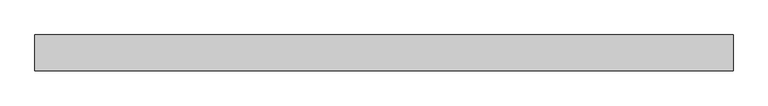
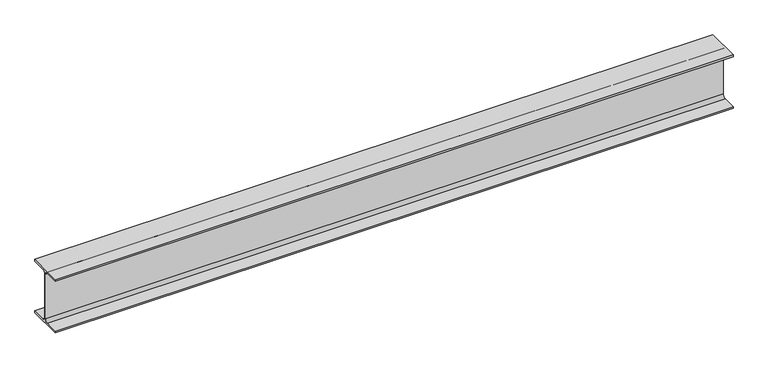
"""IFC4 building model written with IfcOpenShell, lengths in millimetres: beam geometry, 0912_Steel Framing_H-KSD3502 : H_SB_ASB_H-482x300x11x15."""

from ifc_helpers import new_model, si_unit, point, frame, frame_2d, origin, place, context, project, spatial, polyline, circle_curve, trimmed, segment, composite_curve, outline, extrude, source, transform, mapped, element, save


def beam_f33ae538(model_context):
    return source(origin(), model_context, "Body", "SweptSolid", [
        extrude(outline(composite_curve([segment(polyline([(150.0, -226.0), (150.0, -241.0), (-150.0, -241.0), (-150.0, -226.0), (-31.5, -226.0)]), True, "CONTINUOUS"), segment(trimmed(circle_curve(frame_2d((-31.5, -200.0)), 26.0), [point((-31.5, -226.0))], [point((-5.5, -200.0))], True, "CARTESIAN"), True, "CONTINUOUS"), segment(polyline([(-5.5, -200.0), (-5.5, 200.0)]), True, "CONTINUOUS"), segment(trimmed(circle_curve(frame_2d((-31.5, 200.0)), 26.0), [point((-5.5, 200.0))], [point((-31.5, 226.0))], True, "CARTESIAN"), True, "CONTINUOUS"), segment(polyline([(-31.5, 226.0), (-150.0, 226.0), (-150.0, 241.0), (150.0, 241.0), (150.0, 226.0), (31.5, 226.0)]), True, "CONTINUOUS"), segment(trimmed(circle_curve(frame_2d((31.5, 200.0)), 26.0), [point((31.5, 226.0))], [point((5.5, 200.0))], True, "CARTESIAN"), True, "CONTINUOUS"), segment(polyline([(5.5, 200.0), (5.5, -200.0)]), True, "CONTINUOUS"), segment(trimmed(circle_curve(frame_2d((31.5, -200.0)), 26.0), [point((5.5, -200.0))], [point((31.5, -226.0))], True, "CARTESIAN"), True, "CONTINUOUS"), segment(polyline([(31.5, -226.0), (150.0, -226.0)]), True, "CONTINUOUS")], self_intersect=False)), frame((-2904.8, 0.0, 0.0), z_axis=(1.0, 0.0, 0.0), x_axis=(0.0, 1.0, 0.0)), (0.0, 0.0, 1.0), 5809.6),
    ])


if __name__ == "__main__":
    model = new_model("IFC4")
    model_context = context("Model", 3, world=origin())
    ifc_project = project(units=[si_unit("LENGTHUNIT", "METRE", prefix="MILLI")], contexts=[model_context])
    site = spatial("IfcSite", under=ifc_project)
    building = spatial("IfcBuilding", under=site)
    placement = place(None, origin())
    beam_shape = beam_f33ae538(model_context)
    element("IfcBeam", 1, ObjectType="0912_Steel Framing_H-KSD3502 : H_SB_ASB_H-482x300x11x15", at=placement, inside=building, context=model_context, shape_type="MappedRepresentation", body=[
        mapped(beam_shape, transform((0.0, 0.0, 0.0), x_axis=(1.0, 0.0, 0.0), y_axis=(0.0, 1.0, 0.0), z_axis=(0.0, 0.0, 1.0))),
    ])
    save(model, "model.ifc")

# Revit data of these elements
# Type "0912_Steel Framing_H-KSD3502 : H_SB_ASB_H-482x300x11x15"
#   H_WM Code_1 = "S01AA001-00001 | Main Steel Structure Fabrication Work | Shelter/Building | Heavy Steel - Standard (Weight≥90KG/M) | Material: (   )"
#   H_WM Code_2 = "S03AA027-00001 | Main Steel Structure Erection Work | Shelter/Building | Heavy Steel (Weight≥90KG/M) | Material: (   )"
#   H_WM Code_3 = "S01AA010-00001 | Main Steel Structure Fabrication Work | Shelter/Building | Steel Painting/Coating | for Non-Fireproofed Steel Surface, Surface Preparation, Primer, Second & Final Coat | Material: (   )"
#   H_Q'ty Cal Type Tag = "SB-Q2"
#   Width = 30.0 cm
#   Web Thickness = 1.1 cm
#   Web Fillet = 2.6 cm
#   Warping Constant = 3680000.0 cm⁶
#   W = 0
#   Torsional Moment of Inertia = 88.2192 cm⁴
#   Section Area = 145.5 cm²
#   Plastic Modulus weak axis = 695.0 cm³
#   Plastic Modulus strong axis = 2790.0 cm³
#   Perimeter = 2.10 m²/m
#   Nominal Weight = 114.00 kgf/m
#   Moment of Inertia weak axis = 6760.00 cm⁴
#   Moment of Inertia strong axis = 60400.00 cm⁴
#   Height = 48.2 cm
#   Flange Thickness = 1.5 cm
#   Elastic Modulus weak axis = 451.0 cm³
#   Elastic Modulus strong axis = 2500.0 cm³
#   Centroid Vertical = 24.1 cm
#   Centroid Horizontal = 15.0 cm
#   Ix = 604000000
#   Length [instance default] = 1.5240 m
#   Zx = 2790000
#   b = 0.3000 m
#   h = 0.4820 m
#   r = 0.0260 m
#   s = 0.0110 m
#   t = 0.0150 m
#   A = 0.01455 m²
#   Structural Material [instance default] = Steel, 45-345
#   Assembly Code = ""
# Element 1 (IfcBeam, "0912_Steel Framing_H-KSD3502 : H_SB_ASB_H-482x300x11x15")
#   Structural Material = none
# Materials
#   "Steel, 45-345": class "Metal", colour RGB 189 187 185, transparency 0, Description = "Steel 345 MPa", Cost = 0
